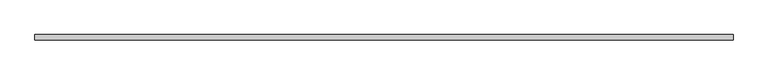
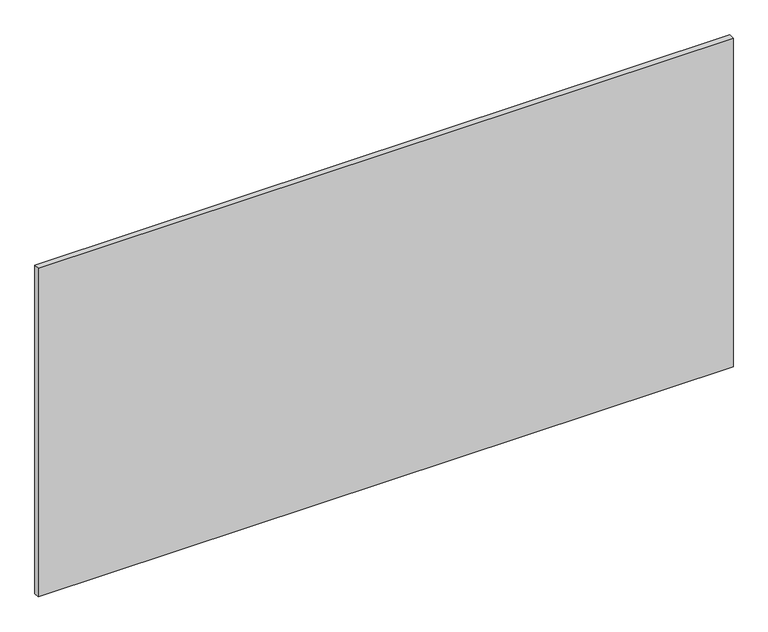
"""IFC4 building model written with IfcOpenShell, lengths in millimetres: proxy geometry, Inner panel:Inner panel:1:Inner panel:1 : Inner panel:Inner panel:300324:300043:Inner panel:1:Inner panel:1 : Inner panel:Inner panel:300324:300043 : Inner panel:Inner panel:1:Inner panel:1 : Inner panel:Inner panel:300324:300043:26 : Inner panel:Inner panel:1:Inner panel:1 : Inner panel:Inner panel:300324:300043:Inner panel:1:Inner panel:1 : Inner panel:Inner panel:300324:300043 : Inner panel:Inner panel:1:Inner panel:1 : Inner panel:Inner panel:300324:300043:300031."""

import ifcopenshell
import ifcopenshell.guid

model = None  # the IFC model being written
_history = None  # IfcOwnerHistory: only IFC2X3 demands one
_inside = {}  # id of a spatial element -> (the spatial element, [elements in it])
_under = {}  # id of a project, library or spatial element -> (it, [spatial elements below it])
_declared = {}  # id of a project -> (the project, [libraries it declares])
_typed = {}  # id of a type object -> (the type object, [elements of that type])
_made_of = {}  # id of a material, layer set ... -> (it, [elements and type objects made of it])


def new_model(schema):
    """Start an empty IFC model of exactly this schema.

    Asked for "IFC4X3", IfcOpenShell would pick the latest addendum, in which some entities
    have other attributes; the version numbers below select the first issue.
    IFC2X3 requires an IfcOwnerHistory on every rooted entity: one is made here for all.
    """
    global model, _history
    if schema == "IFC4X3":
        model = ifcopenshell.file(schema_version=(4, 3, 0, 0))
    else:
        model = ifcopenshell.file(schema=schema)
    _inside.clear()
    _under.clear()
    _declared.clear()
    _typed.clear()
    _made_of.clear()
    _history = None
    if model.schema == "IFC2X3":
        org = make("IfcOrganization", Name="unknown")
        user = make(
            "IfcPersonAndOrganization",
            ThePerson=make("IfcPerson", FamilyName="unknown"),
            TheOrganization=org,
        )
        app = make(
            "IfcApplication",
            ApplicationDeveloper=org,
            Version="unknown",
            ApplicationFullName="unknown",
            ApplicationIdentifier="unknown",
        )
        _history = make(
            "IfcOwnerHistory",
            OwningUser=user,
            OwningApplication=app,
            ChangeAction="ADDED",
            CreationDate=0,
        )
    return model


def make(cls, **values):
    """One entity of the class cls with the attributes given. An attribute that is None is left unset."""
    return model.create_entity(
        cls, **{name: value for name, value in values.items() if value is not None}
    )


def rooted(cls, **values):
    """An entity with a GlobalId (a new one), such as an element, a storey or a relation."""
    return make(cls, GlobalId=ifcopenshell.guid.new(), OwnerHistory=_history, **values)


def si_unit(unit_type, name, prefix=None):
    """IfcSIUnit, for example si_unit("LENGTHUNIT", "METRE", prefix="MILLI")."""
    return make("IfcSIUnit", UnitType=unit_type, Prefix=prefix, Name=name)


def assignment(units):
    """IfcUnitAssignment: the units of a project."""
    return None if units is None else make("IfcUnitAssignment", Units=units)


def point(xyz):
    """IfcCartesianPoint."""
    return None if xyz is None else make("IfcCartesianPoint", Coordinates=xyz)


def direction(xyz):
    """IfcDirection."""
    return None if xyz is None else make("IfcDirection", DirectionRatios=xyz)


def frame(location, z_axis=None, x_axis=None):
    """IfcAxis2Placement3D, a coordinate frame: its origin and axes. An axis left out is left unset."""
    return make(
        "IfcAxis2Placement3D",
        Location=point(location),
        Axis=direction(z_axis),
        RefDirection=direction(x_axis),
    )


def origin():
    """The frame at (0, 0, 0) with its axes left unset."""
    return frame((0.0, 0.0, 0.0))


def place(relative_to, where):
    """IfcLocalPlacement: puts the frame where relative to a parent placement (None: the world)."""
    return make(
        "IfcLocalPlacement", PlacementRelTo=relative_to, RelativePlacement=where
    )


def context(
    kind, dimensions, precision=None, world=None, true_north=None, identifier=None
):
    """IfcGeometricRepresentationContext, for example the 3D "Model" context."""
    return make(
        "IfcGeometricRepresentationContext",
        ContextIdentifier=identifier,
        ContextType=kind,
        CoordinateSpaceDimension=dimensions,
        Precision=precision,
        WorldCoordinateSystem=world,
        TrueNorth=true_north,
    )


def project(units=None, contexts=None):
    """IfcProject with its units and contexts."""
    return rooted(
        "IfcProject",
        Name="project",
        RepresentationContexts=contexts,
        UnitsInContext=assignment(units),
    )


def spatial(cls, under=None, at=None, **own):
    """A site, building, storey or space (cls), placed at a placement, below another one or the project."""
    s = rooted(cls, ObjectPlacement=at, **own)
    if under is not None:
        _under.setdefault(under.id(), (under, []))[1].append(s)
    return s


def polyline(points):
    """IfcPolyline through the points."""
    return make("IfcPolyline", Points=[point(p) for p in points])


def outline(outer, holes=None, kind="AREA"):
    """IfcArbitraryClosedProfileDef: a profile drawn as a closed curve; with holes, ...WithVoids."""
    if holes is None:
        return make("IfcArbitraryClosedProfileDef", ProfileType=kind, OuterCurve=outer)
    return make(
        "IfcArbitraryProfileDefWithVoids",
        ProfileType=kind,
        OuterCurve=outer,
        InnerCurves=holes,
    )


def extrude(swept, where, along, depth):
    """IfcExtrudedAreaSolid: the profile swept, set in the frame where, extruded along a direction by depth."""
    return make(
        "IfcExtrudedAreaSolid",
        SweptArea=swept,
        Position=where,
        ExtrudedDirection=direction(along),
        Depth=depth,
    )


def shape(context_of_items, identifier, shape_type, items):
    """IfcShapeRepresentation: the items that make up one representation, for example the "Body"."""
    return make(
        "IfcShapeRepresentation",
        ContextOfItems=context_of_items,
        RepresentationIdentifier=identifier,
        RepresentationType=shape_type,
        Items=items,
    )


def source(mapping_origin, context_of_items, identifier, shape_type, items):
    """IfcRepresentationMap: a shape defined once, which mapped items show again and again."""
    return make(
        "IfcRepresentationMap",
        MappingOrigin=mapping_origin,
        MappedRepresentation=shape(context_of_items, identifier, shape_type, items),
    )


def transform(
    local_origin,
    x_axis=None,
    y_axis=None,
    z_axis=None,
    scale=None,
    scale2=None,
    scale3=None,
    uniform=True,
):
    """IfcCartesianTransformationOperator3D, or its non-uniform kind. x_axis, y_axis, z_axis: its Axis1, 2, 3."""
    if uniform:
        return make(
            "IfcCartesianTransformationOperator3D",
            Axis1=direction(x_axis),
            Axis2=direction(y_axis),
            LocalOrigin=point(local_origin),
            Scale=scale,
            Axis3=direction(z_axis),
        )
    return make(
        "IfcCartesianTransformationOperator3DnonUniform",
        Axis1=direction(x_axis),
        Axis2=direction(y_axis),
        LocalOrigin=point(local_origin),
        Scale=scale,
        Axis3=direction(z_axis),
        Scale2=scale2,
        Scale3=scale3,
    )


def mapped(mapping_source, mapping_target):
    """IfcMappedItem: shows the shape of a source again, moved by a transform."""
    return make(
        "IfcMappedItem", MappingSource=mapping_source, MappingTarget=mapping_target
    )


def made_of(thing, what):
    """Note that an element or type object is made of a material, layer set ...; save() writes the relation."""
    if what is not None:
        _made_of.setdefault(what.id(), (what, []))[1].append(thing)
    return thing


def element(
    cls,
    number,
    at=None,
    inside=None,
    cuts=None,
    type_object=None,
    material=None,
    context=None,
    identifier="Body",
    shape_type=None,
    held_by="IfcProductDefinitionShape",
    body=None,
    shapes=None,
    **own,
):
    """One element of the class cls, such as IfcWall. Its Tag is "e" and its number.

    at: its placement. inside: the storey or other place that contains it. cuts: it is an
    opening in that element (IfcRelVoidsElement). A single representation is given by context,
    identifier, shape_type and body (its items); several are given by shapes. held_by: the class
    of the entity that holds the representations. save() writes the other relations.
    """
    e = rooted(cls, Tag="e%d" % number, ObjectPlacement=at, **own)
    if body is not None:
        shapes = [shape(context, identifier, shape_type, body)]
    if shapes is not None:
        e.Representation = make(held_by, Representations=shapes)
    if inside is not None:
        _inside.setdefault(inside.id(), (inside, []))[1].append(e)
    if cuts is not None:
        rooted(
            "IfcRelVoidsElement", RelatingBuildingElement=cuts, RelatedOpeningElement=e
        )
    if type_object is not None:
        _typed.setdefault(type_object.id(), (type_object, []))[1].append(e)
    return made_of(e, material)


def aggregate(whole, parts):
    """IfcRelAggregates: a whole, such as a stair, and the parts it consists of."""
    return rooted("IfcRelAggregates", RelatingObject=whole, RelatedObjects=parts)


def save(model, path):
    """Write the relations noted so far, then the file.

    IfcRelAggregates (storeys below a building ...), IfcRelContainedInSpatialStructure (elements
    in a storey), IfcRelDefinesByType, IfcRelAssociatesMaterial and IfcRelDeclares: one each for
    every whole, place, type object, material and project.
    """
    for whole, parts in _under.values():
        aggregate(whole, parts)
    for where, things in _inside.values():
        rooted(
            "IfcRelContainedInSpatialStructure",
            RelatedElements=things,
            RelatingStructure=where,
        )
    for kind, things in _typed.values():
        rooted("IfcRelDefinesByType", RelatedObjects=things, RelatingType=kind)
    for what, things in _made_of.values():
        rooted("IfcRelAssociatesMaterial", RelatedObjects=things, RelatingMaterial=what)
    for by, libraries in _declared.values():
        rooted("IfcRelDeclares", RelatingContext=by, RelatedDefinitions=libraries)
    model.write(path)


def generic_models_3256cd0e(model_context):
    return source(origin(), model_context, "Body", "SweptSolid", [
        extrude(outline(polyline([(590067.7867239, -567913.5913841), (592506.1867239, -567913.5913841), (592506.1867239, -567932.6413841), (590067.7867239, -567932.6413841), (590067.7867239, -567913.5913841)])), frame((0.0, 0.0, 3721.1), z_axis=(0.0, 0.0, 1.0), x_axis=(1.0, 0.0, 0.0)), (0.0, 0.0, 1.0), 1219.2),
    ])


if __name__ == "__main__":
    model = new_model("IFC4")
    model_context = context("Model", 3, world=origin())
    ifc_project = project(units=[si_unit("LENGTHUNIT", "METRE", prefix="MILLI")], contexts=[model_context])
    site = spatial("IfcSite", under=ifc_project)
    building = spatial("IfcBuilding", under=site)
    placement = place(None, origin())
    generic_models_shape = generic_models_3256cd0e(model_context)
    element("IfcBuildingElementProxy", 1, Name="Inner panel:Inner panel:1:Inner panel:1 : Inner panel:Inner panel:300324:300043:Inner panel:1:Inner panel:1 : Inner panel:Inner panel:300324:300043 : Inner panel:Inner panel:1:Inner panel:1 : Inner panel:Inner panel:300324:300043:26 : Inner panel:Inner panel:1:Inner panel:1 : Inner panel:Inner panel:300324:300043:Inner panel:1:Inner panel:1 : Inner panel:Inner panel:300324:300043 : Inner panel:Inner panel:1:Inner panel:1 : Inner panel:Inner panel:300324:300043:300031", ObjectType="Inner panel:Inner panel:1:Inner panel:1 : Inner panel:Inner panel:300324:300043:Inner panel:1:Inner panel:1 : Inner panel:Inner panel:300324:300043 : Inner panel:Inner panel:1:Inner panel:1 : Inner panel:Inner panel:300324:300043:26 : Inner panel:Inner panel:1:Inner panel:1 : Inner panel:Inner panel:300324:300043:Inner panel:1:Inner panel:1 : Inner panel:Inner panel:300324:300043 : Inner panel:Inner panel:1:Inner panel:1 : Inner panel:Inner panel:300324:300043:300031", at=placement, inside=building, context=model_context, shape_type="MappedRepresentation", body=[
        mapped(generic_models_shape, transform((0.0, 0.0, 0.0), x_axis=(1.0, 0.0, 0.0), y_axis=(0.0, 1.0, 0.0), z_axis=(0.0, 0.0, 1.0))),
    ])
    save(model, "model.ifc")

# Revit data of these elements
# Type "Inner panel:Inner panel:1:Inner panel:1 : Inner panel:Inner panel:300324:300043:Inner panel:1:Inner panel:1 : Inner panel:Inner panel:300324:300043 : Inner panel:Inner panel:1:Inner panel:1 : Inner panel:Inner panel:300324:300043:26 : Inner panel:Inner panel:1:Inner panel:1 : Inner panel:Inner panel:300324:300043:Inner panel:1:Inner panel:1 : Inner panel:Inner panel:300324:300043 : Inner panel:Inner panel:1:Inner panel:1 : Inner panel:Inner panel:300324:300043:300031"
#   NameOverride = "Inner panel:Inner panel:1:Inner panel:1 : Inner panel:Inner panel:300324:300043:Inner panel:1:Inner panel:1 : Inner panel:Inner panel:300324:300043 : Inner panel:Inner panel:1:Inner panel:1 : Inner panel:Inner panel:300324:300043:300031"
#   ObjectTypeOverride = "Inner panel:1:Inner panel:1 : Inner panel:Inner panel:300324:300043 : Inner panel:Inner panel:1:Inner panel:1 : Inner panel:Inner panel:300324:300043"
#   Reference = "Inner panel"
#   Tag = "300031"
# Element 1 (IfcBuildingElementProxy, "Inner panel:Inner panel:1:Inner panel:1 : Inner panel:Inner panel:300324:300043:Inner panel:1:Inner panel:1 : Inner panel:Inner panel:300324:300043 : Inner panel:Inner panel:1:Inner panel:1 : Inner panel:Inner panel:300324:300043:26 : Inner panel:Inner panel:1:Inner panel:1 : Inner panel:Inner panel:300324:300043:Inner panel:1:Inner panel:1 : Inner panel:Inner panel:300324:300043 : Inner panel:Inner panel:1:Inner panel:1 : Inner panel:Inner panel:300324:300043:300031")
#   Materials on its faces: "3/4\" PREFINISHED STAINED/SEALED PLYWOOD (FINISH: GRADE B,  FLAME SPREAD: CLASS B)"
# Materials
#   "3/4\" PREFINISHED STAINED/SEALED PLYWOOD (FINISH: GRADE B,  FLAME SPREAD: CLASS B)": class "Wood", colour RGB 149 120 74, transparency 0, Description = "Plywood, sheathing grade", Cost = 0
